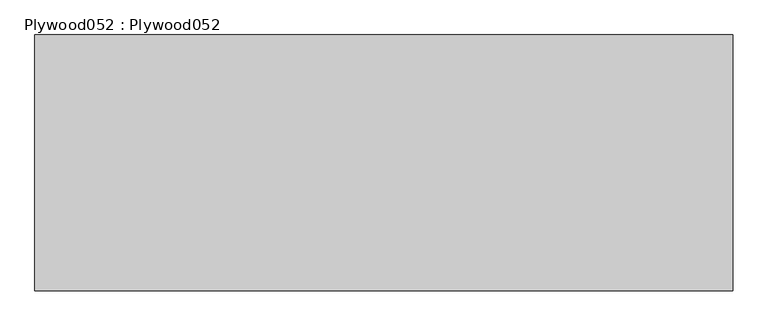
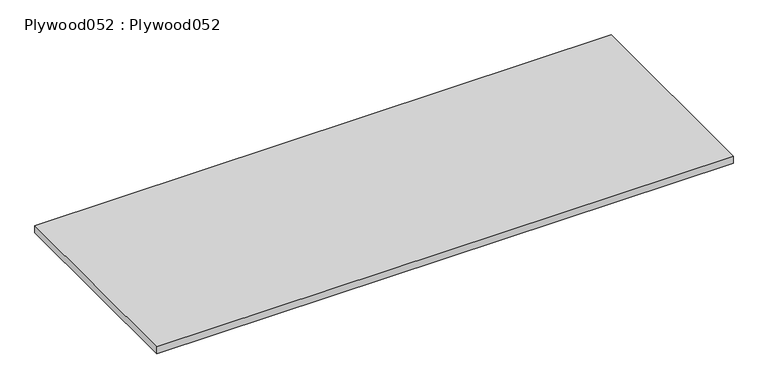
"""IFC4 building model written with IfcOpenShell, lengths in millimetres: proxy geometry, Plywood052 : Plywood052."""

from ifc_helpers import new_model, si_unit, frame, origin, place, context, project, spatial, polyline, outline, extrude, source, transform, mapped, element, save


def plywood052_plywood052_1b8d1a6a(model_context):
    return source(origin(), model_context, "Body", "SweptSolid", [
        extrude(outline(polyline([(14383.0178845, -3764.4167972), (14383.0178845, -4497.8417972), (12383.0178845, -4497.8417972), (12383.0178845, -3764.4167972), (14383.0178845, -3764.4167972)])), frame((0.0, 0.0, 36531.296), z_axis=(0.0, 0.0, 1.0), x_axis=(1.0, 0.0, 0.0)), (0.0, 0.0, 1.0), 25.4),
    ])


if __name__ == "__main__":
    model = new_model("IFC4")
    model_context = context("Model", 3, world=origin())
    ifc_project = project(units=[si_unit("LENGTHUNIT", "METRE", prefix="MILLI")], contexts=[model_context])
    site = spatial("IfcSite", under=ifc_project)
    building = spatial("IfcBuilding", under=site)
    placement = place(None, origin())
    plywood052_plywood052_shape = plywood052_plywood052_1b8d1a6a(model_context)
    element("IfcBuildingElementProxy", 1, Name="Plywood052 : Plywood052", ObjectType="Plywood052 : Plywood052", at=placement, inside=building, context=model_context, shape_type="MappedRepresentation", body=[
        mapped(plywood052_plywood052_shape, transform((0.0, 0.0, 0.0), x_axis=(1.0, 0.0, 0.0), y_axis=(0.0, 1.0, 0.0), z_axis=(0.0, 0.0, 1.0))),
    ])
    save(model, "model.ifc")

# Revit data of these elements
# Type "Plywood052 : Plywood052"
#   NameOverride = "Plywood052"
# Element 1 (IfcBuildingElementProxy, "Plywood052 : Plywood052")
#   Materials on its faces: "3/4\" TREATED CDX PLYWOOD OVER 6 MIL POLYETHYLENE VAPOR BARRIER"
# Materials
#   "3/4\" TREATED CDX PLYWOOD OVER 6 MIL POLYETHYLENE VAPOR BARRIER": class "Unassigned", colour RGB 67 103 56, transparency 0, Cost = 0
